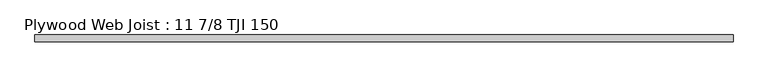
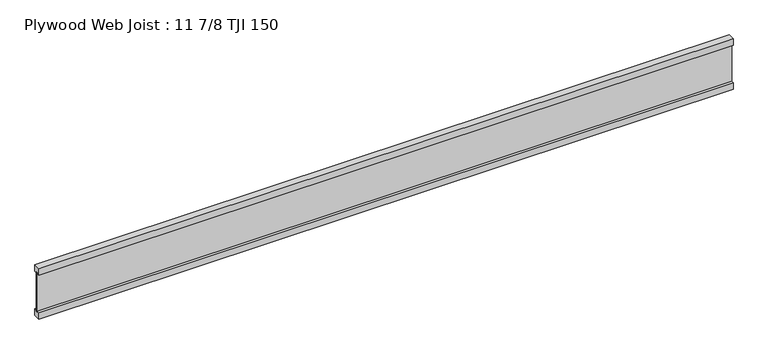
"""IFC4 building model written with IfcOpenShell, lengths in millimetres: beam geometry, Plywood Web Joist : 11 7/8 TJI 150."""

from ifc_helpers import new_model, si_unit, frame, origin, place, context, project, spatial, polyline, outline, extrude, source, transform, mapped, element, save


def plywood_web_joist_11_7_8_tji_150_4ba6f87f(model_context):
    return source(origin(), model_context, "Body", "SweptSolid", [
        extrude(outline(polyline([(-19.05, 150.8125), (19.05, 150.8125), (19.05, 112.7125), (4.7625, 112.7125), (4.7625, 119.0625), (-4.7625, 119.0625), (-4.7625, 112.7125), (-19.05, 112.7125), (-19.05, 150.8125)])), frame((-1967.70625, 0.0, 0.0), z_axis=(1.0, 0.0, 0.0), x_axis=(0.0, 1.0, 0.0)), (0.0, 0.0, 1.0), 3935.4125),
        extrude(outline(polyline([(19.05, -112.7125), (19.05, -150.8125), (-19.05, -150.8125), (-19.05, -112.7125), (-4.7625, -112.7125), (-4.7625, -118.3285374), (4.7625, -118.3285374), (4.7625, -112.7125), (19.05, -112.7125)])), frame((-1967.70625, 0.0, 0.0), z_axis=(1.0, 0.0, 0.0), x_axis=(0.0, 1.0, 0.0)), (0.0, 0.0, 1.0), 3935.4125),
        extrude(outline(polyline([(1967.70625, 4.7625), (1967.70625, -4.7625), (-1967.70625, -4.7625), (-1967.70625, 4.7625), (1967.70625, 4.7625)])), frame((0.0, 0.0, -118.3285374), z_axis=(0.0, 0.0, 1.0), x_axis=(1.0, 0.0, 0.0)), (0.0, 0.0, 1.0), 237.3910374),
    ])


if __name__ == "__main__":
    model = new_model("IFC4")
    model_context = context("Model", 3, world=origin())
    ifc_project = project(units=[si_unit("LENGTHUNIT", "METRE", prefix="MILLI")], contexts=[model_context])
    site = spatial("IfcSite", under=ifc_project)
    building = spatial("IfcBuilding", under=site)
    placement = place(None, origin())
    plywood_web_joist_11_7_8_tji_150_shape = plywood_web_joist_11_7_8_tji_150_4ba6f87f(model_context)
    element("IfcBeam", 1, ObjectType="Plywood Web Joist : 11 7/8 TJI 150", at=placement, inside=building, context=model_context, shape_type="MappedRepresentation", body=[
        mapped(plywood_web_joist_11_7_8_tji_150_shape, transform((0.0, 0.0, 0.0), x_axis=(1.0, 0.0, 0.0), y_axis=(0.0, 1.0, 0.0), z_axis=(0.0, 0.0, 1.0))),
    ])
    save(model, "model.ifc")

# Revit data of these elements
# Type "Plywood Web Joist : 11 7/8 TJI 150"
#   Assembly Code = "B10"
#   Cost = 17.5
#   Length [instance default] = 5' - 0"
#   b = 0' - 1 1/2"
#   d = 0' - 11 7/8"
#   Structural Material [instance default] = Softwood, Lumber
# Element 1 (IfcBeam, "Plywood Web Joist : 11 7/8 TJI 150")
#   Structural Material = Douglas Fir #2
#   Materials on its faces: "Douglas Fir #2"
# Materials
#   "Softwood, Lumber": class "Wood", colour RGB 223 192 134, transparency 0, Description = "Pinus Echinata", Cost = 0
#   "Douglas Fir #2": class "Wood", colour RGB 223 192 134, transparency 0, Description = "Pinus Echinata", Cost = 0
